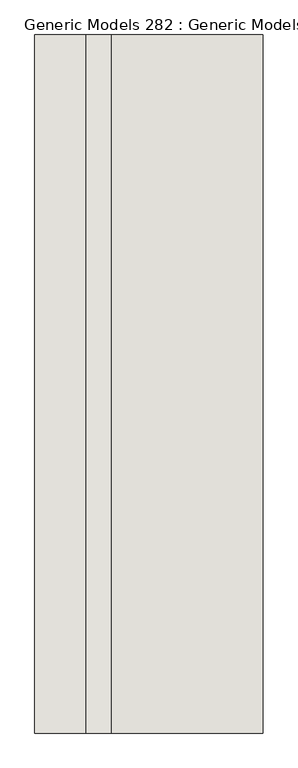
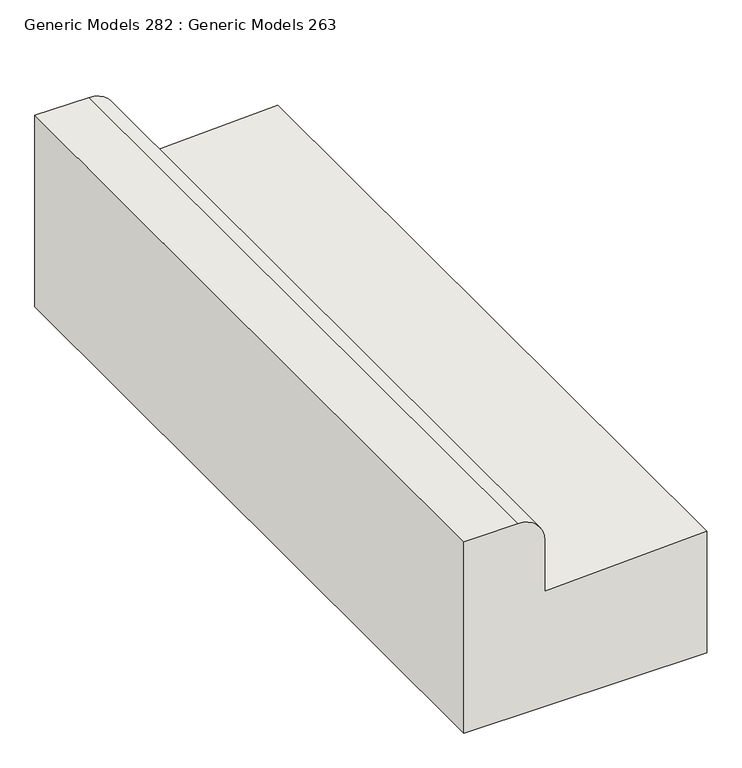
"""IFC4 building model written with IfcOpenShell, lengths in millimetres: wall geometry, Generic Models 282 : Generic Models 263."""

from ifc_helpers import new_model, si_unit, point, frame, frame_2d, origin, place, context, project, spatial, polyline, circle_curve, trimmed, segment, composite_curve, outline, extrude, source, transform, mapped, element, save


def generic_models_282_generic_models_263_cc0d5e36(model_context):
    return source(origin(), model_context, "Body", "SweptSolid", [
        extrude(outline(composite_curve([segment(polyline([(0.0, 91681.5797726), (0.0, 91579.9797726), (-381.0, 91579.9797726), (-381.0, 92037.1797726), (-139.7, 92037.1797726), (-152.4, 91732.3797726), (-50.8, 91732.3797726)]), True, "CONTINUOUS"), segment(trimmed(circle_curve(frame_2d((-50.8, 91681.5797726)), 50.8), [point((-50.8, 91732.3797726))], [point((0.0, 91681.5797726))], False, "CARTESIAN"), True, "CONTINUOUS")], self_intersect=False)), frame((0.0, 2106.5727422, 0.0), z_axis=(0.0, 1.0, 0.0), x_axis=(0.0, 0.0, 1.0)), (0.0, 0.0, 1.0), 1397.4322547),
    ])


if __name__ == "__main__":
    model = new_model("IFC4")
    model_context = context("Model", 3, world=origin())
    ifc_project = project(units=[si_unit("LENGTHUNIT", "METRE", prefix="MILLI")], contexts=[model_context])
    site = spatial("IfcSite", under=ifc_project)
    building = spatial("IfcBuilding", under=site)
    placement = place(None, origin())
    generic_models_282_generic_models_263_shape = generic_models_282_generic_models_263_cc0d5e36(model_context)
    element("IfcWall", 1, ObjectType="Generic Models 282 : Generic Models 263", at=placement, inside=building, context=model_context, shape_type="MappedRepresentation", body=[
        mapped(generic_models_282_generic_models_263_shape, transform((0.0, 0.0, 0.0), x_axis=(1.0, 0.0, 0.0), y_axis=(0.0, 1.0, 0.0), z_axis=(0.0, 0.0, 1.0))),
    ])
    save(model, "model.ifc")

# Revit data of these elements
# Element 1 (IfcWall, "Generic Models 282 : Generic Models 263")
#   Materials on its faces: "CONCRETE CURB"
# Materials
#   "CONCRETE CURB": class "Concrete", colour RGB 191 191 191, transparency 0, Description = "Cast-in-place concrete", Cost = 0
